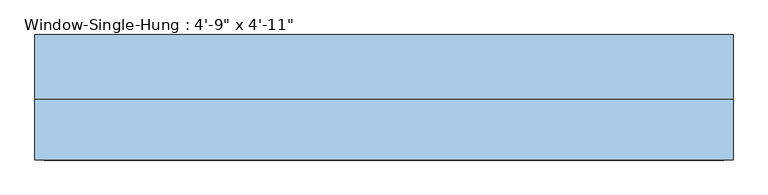
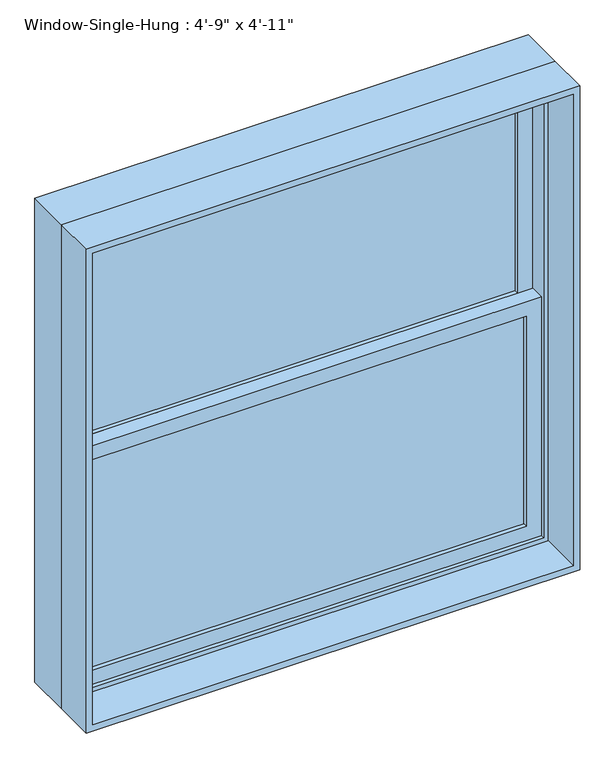
"""IFC4 building model written with IfcOpenShell, lengths in millimetres: window geometry."""

from ifc_helpers import new_model, si_unit, frame, origin, place, context, project, spatial, polyline, outline, extrude, source, transform, mapped, element, save


def window_55bfdad2(model_context):
    return source(origin(), model_context, "Body", "SweptSolid", [
        extrude(outline(polyline([(647.7, 50.8), (647.7, 44.45), (-647.7, 44.45), (-647.7, 50.8), (647.7, 50.8)])), frame((0.0, 0.0, 990.6), z_axis=(0.0, 0.0, 1.0), x_axis=(1.0, 0.0, 0.0)), (0.0, 0.0, 1.0), 650.875),
        extrude(outline(polyline([(-647.7, 38.1), (647.7, 38.1), (647.7, 31.75), (-647.7, 31.75), (-647.7, 38.1)])), frame((0.0, 0.0, 990.6), z_axis=(0.0, 0.0, 1.0), x_axis=(1.0, 0.0, 0.0)), (0.0, 0.0, 1.0), 650.875),
        extrude(outline(polyline([(647.7, 95.25), (647.7, 88.9), (-647.7, 88.9), (-647.7, 95.25), (647.7, 95.25)])), frame((0.0, 0.0, 1685.925), z_axis=(0.0, 0.0, 1.0), x_axis=(1.0, 0.0, 0.0)), (0.0, 0.0, 1.0), 650.875),
        extrude(outline(polyline([(-647.7, 82.55), (647.7, 82.55), (647.7, 76.2), (-647.7, 76.2), (-647.7, 82.55)])), frame((0.0, 0.0, 1685.925), z_axis=(0.0, 0.0, 1.0), x_axis=(1.0, 0.0, 0.0)), (0.0, 0.0, 1.0), 650.875),
        extrude(outline(polyline([(1685.925, -692.15), (946.15, -692.15), (946.15, 692.15), (1685.925, 692.15), (1685.925, -692.15)]), holes=[polyline([(1641.475, 647.7), (990.6, 647.7), (990.6, -647.7), (1641.475, -647.7), (1641.475, 647.7)])]), frame((0.0, 19.05, 0.0), z_axis=(0.0, 1.0, 0.0), x_axis=(0.0, 0.0, 1.0)), (0.0, 0.0, 1.0), 44.45),
        extrude(outline(polyline([(2381.25, -692.15), (1641.475, -692.15), (1641.475, 692.15), (2381.25, 692.15), (2381.25, -692.15)]), holes=[polyline([(2336.8, 647.7), (1685.925, 647.7), (1685.925, -647.7), (2336.8, -647.7), (2336.8, 647.7)])]), frame((0.0, 63.5, 0.0), z_axis=(0.0, 1.0, 0.0), x_axis=(0.0, 0.0, 1.0)), (0.0, 0.0, 1.0), 44.45),
        extrude(outline(polyline([(2413.0, -723.9), (914.4, -723.9), (914.4, 723.9), (2413.0, 723.9), (2413.0, -723.9)]), holes=[polyline([(2381.25, 692.15), (946.15, 692.15), (946.15, -692.15), (2381.25, -692.15), (2381.25, 692.15)])]), frame((0.0, 6.35, 0.0), z_axis=(0.0, 1.0, 0.0), x_axis=(0.0, 0.0, 1.0)), (0.0, 0.0, 1.0), 133.35),
        extrude(outline(polyline([(2413.0, 723.9), (2413.0, -723.9), (914.4, -723.9), (914.4, 723.9), (2413.0, 723.9)]), holes=[polyline([(2393.95, 704.85), (933.45, 704.85), (933.45, -704.85), (2393.95, -704.85), (2393.95, 704.85)])]), frame((0.0, -120.65, 0.0), z_axis=(0.0, 1.0, 0.0), x_axis=(0.0, 0.0, 1.0)), (0.0, 0.0, 1.0), 127.0),
    ])


if __name__ == "__main__":
    model = new_model("IFC4")
    model_context = context("Model", 3, world=origin())
    ifc_project = project(units=[si_unit("LENGTHUNIT", "METRE", prefix="MILLI")], contexts=[model_context])
    site = spatial("IfcSite", under=ifc_project)
    building = spatial("IfcBuilding", under=site)
    placement = place(None, origin())
    window_shape = window_55bfdad2(model_context)
    element("IfcWindow", 1, ObjectType="Window-Single-Hung : 4'-9\" x 4'-11\"", at=placement, inside=building, context=model_context, shape_type="MappedRepresentation", body=[
        mapped(window_shape, transform((0.0, 0.0, 0.0), x_axis=(1.0, 0.0, 0.0), y_axis=(0.0, 1.0, 0.0), z_axis=(0.0, 0.0, 1.0))),
    ])
    save(model, "model.ifc")

# Revit data of these elements
# Type "Window-Single-Hung : 4'-9\" x 4'-11\""
#   Type Mark = "23"
#   Fire Rating = "0.5h"
#   Construction Type Id = "DG-DR"
#   Assembly Code = "B2020100"
#   Analytic Construction = "Double glazing - domestic"
#   Wall Thickness [instance default] = 0' - 6"
#   Window Inset [instance default] = 0' - 0"
#   Visual Light Transmittance = 0.81
#   Thermal Resistance (R) = 0.319569 (m²·K)/W
#   Solar Heat Gain Coefficient = 0.76
#   Muntin Width = 4' - 3"
#   Muntin Height = 2' - 1 5/8"
#   Interior Wall Closure [instance default] = 0' - 1 1/2"
#   Rough Width = 4' - 9 1/2"
#   Rough Height = 4' - 11 1/2"
#   Frame Extension [instance default] = 0' - 1 1/4"
#   Exterior Wall Closure [instance default] = 0' - 0 1/2"
#   Extension Jamb [instance default] = 0' - 1 1/2"
#   Heat Transfer Coefficient (U) = 3.12929 W/(m²·K)
#   Height = 4' - 11"
#   Width = 4' - 9"
#   Top Muntin Visibility = no
#   Indicator Visibility = no
#   Extension Jamb Visibility [instance default] = yes
#   Interior Trim Visibility [instance default] = yes
#   Exterior Trim Visibility [instance default] = yes
#   Bottom Muntin Visibility = no
#   Muntin Pattern = Muntin Pattern_2x2 : Muntin Pattern_2x2
#   Interior Trim Material = Wood - Stained
#   Interior Trim = Trim-Window-Interior-Flat : Picture Frame
#   Exterior Trim Material = Clad - White
#   Exterior Trim = Trim-Window-Exterior-Flat : with Sill
#   Glass Panel Material = Glass
#   Exterior Frame Material = Clad - White
#   Interior Frame Material = Wood - Stained
#   Wall Closure = (empty or 0)
# Element 1 (IfcWindow, "Window-Single-Hung : 4'-9\" x 4'-11\"")
#   Wall Thickness = 0' - 9 1/2"
#   Extension Jamb = 0' - 5"
#   Materials on its faces: "Wood - Stained", "Glass", "Clad - White"
# Materials
#   "Wood - Stained": class "Wood", colour RGB 224 178 126, transparency 0, Cost = 0
#   "Clad - White": class "Wood", colour RGB 242 242 238, transparency 0, Cost = 0
#   "Glass": class "Glass", colour RGB 218 227 224, transparency 0.85, Description = "Soda Lime Glass", Cost = 0
